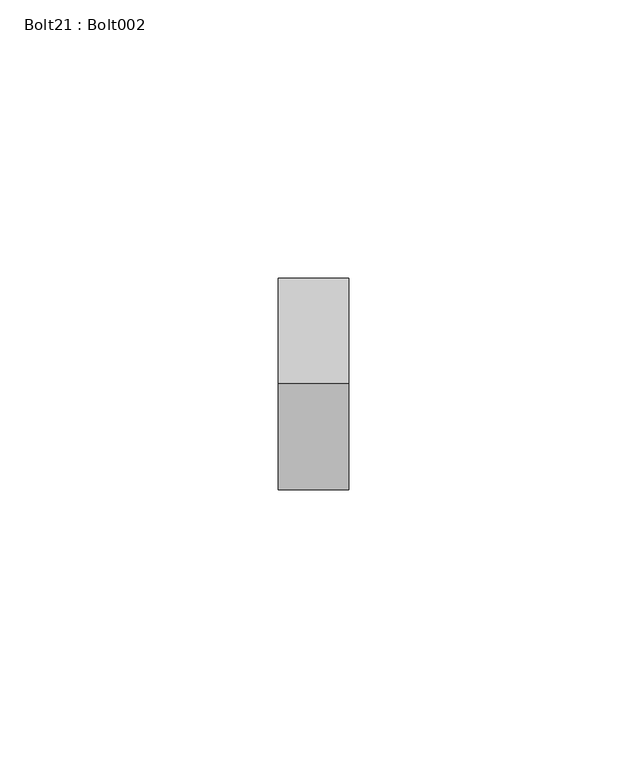
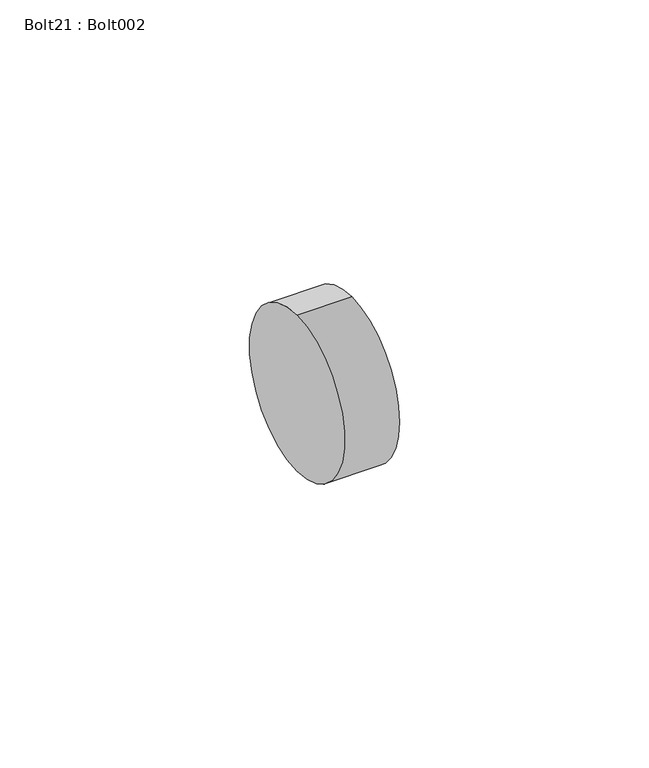
"""IFC4 building model written with IfcOpenShell, lengths in millimetres: proxy geometry, Bolt21 : Bolt002."""

import ifcopenshell
import ifcopenshell.guid

model = None  # the IFC model being written
_history = None  # IfcOwnerHistory: only IFC2X3 demands one
_inside = {}  # id of a spatial element -> (the spatial element, [elements in it])
_under = {}  # id of a project, library or spatial element -> (it, [spatial elements below it])
_declared = {}  # id of a project -> (the project, [libraries it declares])
_typed = {}  # id of a type object -> (the type object, [elements of that type])
_made_of = {}  # id of a material, layer set ... -> (it, [elements and type objects made of it])


def new_model(schema):
    """Start an empty IFC model of exactly this schema.

    Asked for "IFC4X3", IfcOpenShell would pick the latest addendum, in which some entities
    have other attributes; the version numbers below select the first issue.
    IFC2X3 requires an IfcOwnerHistory on every rooted entity: one is made here for all.
    """
    global model, _history
    if schema == "IFC4X3":
        model = ifcopenshell.file(schema_version=(4, 3, 0, 0))
    else:
        model = ifcopenshell.file(schema=schema)
    _inside.clear()
    _under.clear()
    _declared.clear()
    _typed.clear()
    _made_of.clear()
    _history = None
    if model.schema == "IFC2X3":
        org = make("IfcOrganization", Name="unknown")
        user = make(
            "IfcPersonAndOrganization",
            ThePerson=make("IfcPerson", FamilyName="unknown"),
            TheOrganization=org,
        )
        app = make(
            "IfcApplication",
            ApplicationDeveloper=org,
            Version="unknown",
            ApplicationFullName="unknown",
            ApplicationIdentifier="unknown",
        )
        _history = make(
            "IfcOwnerHistory",
            OwningUser=user,
            OwningApplication=app,
            ChangeAction="ADDED",
            CreationDate=0,
        )
    return model


def make(cls, **values):
    """One entity of the class cls with the attributes given. An attribute that is None is left unset."""
    return model.create_entity(
        cls, **{name: value for name, value in values.items() if value is not None}
    )


def rooted(cls, **values):
    """An entity with a GlobalId (a new one), such as an element, a storey or a relation."""
    return make(cls, GlobalId=ifcopenshell.guid.new(), OwnerHistory=_history, **values)


def si_unit(unit_type, name, prefix=None):
    """IfcSIUnit, for example si_unit("LENGTHUNIT", "METRE", prefix="MILLI")."""
    return make("IfcSIUnit", UnitType=unit_type, Prefix=prefix, Name=name)


def assignment(units):
    """IfcUnitAssignment: the units of a project."""
    return None if units is None else make("IfcUnitAssignment", Units=units)


def point(xyz):
    """IfcCartesianPoint."""
    return None if xyz is None else make("IfcCartesianPoint", Coordinates=xyz)


def direction(xyz):
    """IfcDirection."""
    return None if xyz is None else make("IfcDirection", DirectionRatios=xyz)


def frame(location, z_axis=None, x_axis=None):
    """IfcAxis2Placement3D, a coordinate frame: its origin and axes. An axis left out is left unset."""
    return make(
        "IfcAxis2Placement3D",
        Location=point(location),
        Axis=direction(z_axis),
        RefDirection=direction(x_axis),
    )


def frame_2d(location, x_axis=None):
    """IfcAxis2Placement2D, a coordinate frame in the plane: its origin and x axis."""
    return make(
        "IfcAxis2Placement2D", Location=point(location), RefDirection=direction(x_axis)
    )


def origin():
    """The frame at (0, 0, 0) with its axes left unset."""
    return frame((0.0, 0.0, 0.0))


def place(relative_to, where):
    """IfcLocalPlacement: puts the frame where relative to a parent placement (None: the world)."""
    return make(
        "IfcLocalPlacement", PlacementRelTo=relative_to, RelativePlacement=where
    )


def context(
    kind, dimensions, precision=None, world=None, true_north=None, identifier=None
):
    """IfcGeometricRepresentationContext, for example the 3D "Model" context."""
    return make(
        "IfcGeometricRepresentationContext",
        ContextIdentifier=identifier,
        ContextType=kind,
        CoordinateSpaceDimension=dimensions,
        Precision=precision,
        WorldCoordinateSystem=world,
        TrueNorth=true_north,
    )


def project(units=None, contexts=None):
    """IfcProject with its units and contexts."""
    return rooted(
        "IfcProject",
        Name="project",
        RepresentationContexts=contexts,
        UnitsInContext=assignment(units),
    )


def spatial(cls, under=None, at=None, **own):
    """A site, building, storey or space (cls), placed at a placement, below another one or the project."""
    s = rooted(cls, ObjectPlacement=at, **own)
    if under is not None:
        _under.setdefault(under.id(), (under, []))[1].append(s)
    return s


def circle_curve(where, radius):
    """IfcCircle in the frame where."""
    return make("IfcCircle", Position=where, Radius=radius)


def trimmed(basis, trim1, trim2, sense, master):
    """IfcTrimmedCurve: the piece of a basis curve between two trims."""
    return make(
        "IfcTrimmedCurve",
        BasisCurve=basis,
        Trim1=trim1,
        Trim2=trim2,
        SenseAgreement=sense,
        MasterRepresentation=master,
    )


def segment(curve, same_sense, transition):
    """IfcCompositeCurveSegment."""
    return make(
        "IfcCompositeCurveSegment",
        Transition=transition,
        SameSense=same_sense,
        ParentCurve=curve,
    )


def composite_curve(segments, self_intersect=None):
    """IfcCompositeCurve: segments joined end to end."""
    return make("IfcCompositeCurve", Segments=segments, SelfIntersect=self_intersect)


def outline(outer, holes=None, kind="AREA"):
    """IfcArbitraryClosedProfileDef: a profile drawn as a closed curve; with holes, ...WithVoids."""
    if holes is None:
        return make("IfcArbitraryClosedProfileDef", ProfileType=kind, OuterCurve=outer)
    return make(
        "IfcArbitraryProfileDefWithVoids",
        ProfileType=kind,
        OuterCurve=outer,
        InnerCurves=holes,
    )


def extrude(swept, where, along, depth):
    """IfcExtrudedAreaSolid: the profile swept, set in the frame where, extruded along a direction by depth."""
    return make(
        "IfcExtrudedAreaSolid",
        SweptArea=swept,
        Position=where,
        ExtrudedDirection=direction(along),
        Depth=depth,
    )


def shape(context_of_items, identifier, shape_type, items):
    """IfcShapeRepresentation: the items that make up one representation, for example the "Body"."""
    return make(
        "IfcShapeRepresentation",
        ContextOfItems=context_of_items,
        RepresentationIdentifier=identifier,
        RepresentationType=shape_type,
        Items=items,
    )


def source(mapping_origin, context_of_items, identifier, shape_type, items):
    """IfcRepresentationMap: a shape defined once, which mapped items show again and again."""
    return make(
        "IfcRepresentationMap",
        MappingOrigin=mapping_origin,
        MappedRepresentation=shape(context_of_items, identifier, shape_type, items),
    )


def transform(
    local_origin,
    x_axis=None,
    y_axis=None,
    z_axis=None,
    scale=None,
    scale2=None,
    scale3=None,
    uniform=True,
):
    """IfcCartesianTransformationOperator3D, or its non-uniform kind. x_axis, y_axis, z_axis: its Axis1, 2, 3."""
    if uniform:
        return make(
            "IfcCartesianTransformationOperator3D",
            Axis1=direction(x_axis),
            Axis2=direction(y_axis),
            LocalOrigin=point(local_origin),
            Scale=scale,
            Axis3=direction(z_axis),
        )
    return make(
        "IfcCartesianTransformationOperator3DnonUniform",
        Axis1=direction(x_axis),
        Axis2=direction(y_axis),
        LocalOrigin=point(local_origin),
        Scale=scale,
        Axis3=direction(z_axis),
        Scale2=scale2,
        Scale3=scale3,
    )


def mapped(mapping_source, mapping_target):
    """IfcMappedItem: shows the shape of a source again, moved by a transform."""
    return make(
        "IfcMappedItem", MappingSource=mapping_source, MappingTarget=mapping_target
    )


def made_of(thing, what):
    """Note that an element or type object is made of a material, layer set ...; save() writes the relation."""
    if what is not None:
        _made_of.setdefault(what.id(), (what, []))[1].append(thing)
    return thing


def element(
    cls,
    number,
    at=None,
    inside=None,
    cuts=None,
    type_object=None,
    material=None,
    context=None,
    identifier="Body",
    shape_type=None,
    held_by="IfcProductDefinitionShape",
    body=None,
    shapes=None,
    **own,
):
    """One element of the class cls, such as IfcWall. Its Tag is "e" and its number.

    at: its placement. inside: the storey or other place that contains it. cuts: it is an
    opening in that element (IfcRelVoidsElement). A single representation is given by context,
    identifier, shape_type and body (its items); several are given by shapes. held_by: the class
    of the entity that holds the representations. save() writes the other relations.
    """
    e = rooted(cls, Tag="e%d" % number, ObjectPlacement=at, **own)
    if body is not None:
        shapes = [shape(context, identifier, shape_type, body)]
    if shapes is not None:
        e.Representation = make(held_by, Representations=shapes)
    if inside is not None:
        _inside.setdefault(inside.id(), (inside, []))[1].append(e)
    if cuts is not None:
        rooted(
            "IfcRelVoidsElement", RelatingBuildingElement=cuts, RelatedOpeningElement=e
        )
    if type_object is not None:
        _typed.setdefault(type_object.id(), (type_object, []))[1].append(e)
    return made_of(e, material)


def aggregate(whole, parts):
    """IfcRelAggregates: a whole, such as a stair, and the parts it consists of."""
    return rooted("IfcRelAggregates", RelatingObject=whole, RelatedObjects=parts)


def save(model, path):
    """Write the relations noted so far, then the file.

    IfcRelAggregates (storeys below a building ...), IfcRelContainedInSpatialStructure (elements
    in a storey), IfcRelDefinesByType, IfcRelAssociatesMaterial and IfcRelDeclares: one each for
    every whole, place, type object, material and project.
    """
    for whole, parts in _under.values():
        aggregate(whole, parts)
    for where, things in _inside.values():
        rooted(
            "IfcRelContainedInSpatialStructure",
            RelatedElements=things,
            RelatingStructure=where,
        )
    for kind, things in _typed.values():
        rooted("IfcRelDefinesByType", RelatedObjects=things, RelatingType=kind)
    for what, things in _made_of.values():
        rooted("IfcRelAssociatesMaterial", RelatedObjects=things, RelatingMaterial=what)
    for by, libraries in _declared.values():
        rooted("IfcRelDeclares", RelatingContext=by, RelatedDefinitions=libraries)
    model.write(path)


def bolt21_bolt002_beea302d(model_context):
    return source(origin(), model_context, "Body", "SweptSolid", [
        extrude(outline(composite_curve([segment(trimmed(circle_curve(frame_2d((1985.8304801, 40070.0545241)), 19.05), [point((1985.8304801, 40051.0045241))], [point((1985.8304801, 40089.1045241))], False, "CARTESIAN"), True, "CONTINUOUS"), segment(trimmed(circle_curve(frame_2d((1985.8304801, 40070.0545241)), 19.05), [point((1985.8304801, 40089.1045241))], [point((1985.8304801, 40051.0045241))], False, "CARTESIAN"), True, "CONTINUOUS")], self_intersect=False)), frame((10268.2640809, 0.0, 0.0), z_axis=(1.0, 0.0, 0.0), x_axis=(0.0, 1.0, 0.0)), (0.0, 0.0, 1.0), 12.7),
    ])


if __name__ == "__main__":
    model = new_model("IFC4")
    model_context = context("Model", 3, world=origin())
    ifc_project = project(units=[si_unit("LENGTHUNIT", "METRE", prefix="MILLI")], contexts=[model_context])
    site = spatial("IfcSite", under=ifc_project)
    building = spatial("IfcBuilding", under=site)
    placement = place(None, origin())
    bolt21_bolt002_shape = bolt21_bolt002_beea302d(model_context)
    element("IfcBuildingElementProxy", 1, Name="Bolt21 : Bolt002", ObjectType="Bolt21 : Bolt002", at=placement, inside=building, context=model_context, shape_type="MappedRepresentation", body=[
        mapped(bolt21_bolt002_shape, transform((0.0, 0.0, 0.0), x_axis=(1.0, 0.0, 0.0), y_axis=(0.0, 1.0, 0.0), z_axis=(0.0, 0.0, 1.0))),
    ])
    save(model, "model.ifc")

# Revit data of these elements
# Type "Bolt21 : Bolt002"
#   NameOverride = "Bolt002"
# Element 1 (IfcBuildingElementProxy, "Bolt21 : Bolt002")
#   Materials on its faces: "TUBE STEEL STRINGER WELDED TO ANCHORED STEEL PLATE - SEE STRUCT DWGS"
# Materials
#   "TUBE STEEL STRINGER WELDED TO ANCHORED STEEL PLATE - SEE STRUCT DWGS": class "Unassigned", colour RGB 128 128 128, transparency 0, Cost = 0
